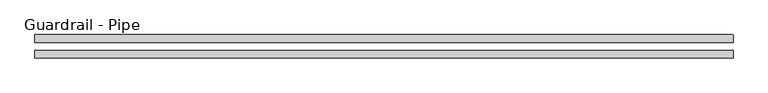
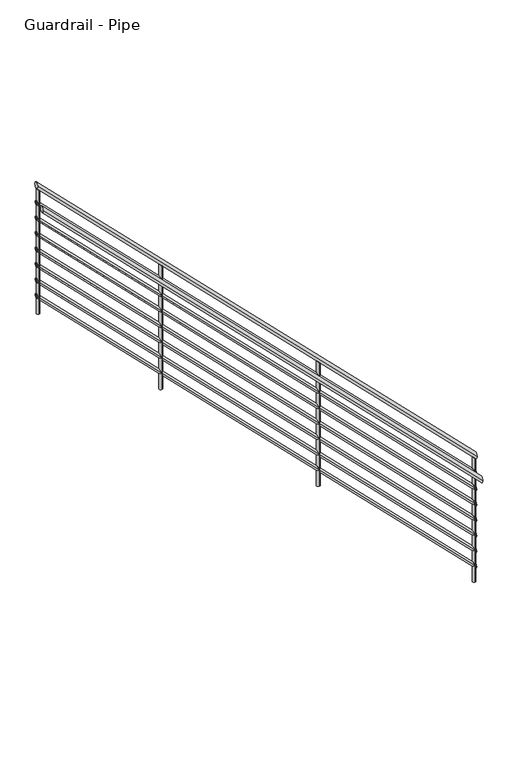
"""IFC4 building model written with IfcOpenShell, lengths in millimetres: railing geometry, Guardrail - Pipe."""

from ifc_helpers import new_model, si_unit, frame, origin, place, context, project, spatial, circle_curve, ellipse_curve, source, transform, mapped, element, save
from ifc_brep_helpers import plane_surface, cylinder_surface, advanced_brep


def guardrail_pipe_ce189c05(model_context):
    return source(origin(), model_context, "Body", "AdvancedBrep", [
        advanced_brep(
        [(-7243.3085296, -3994.9836772, 1268.4592316), (-7243.3085296, -3956.8836772, 1268.4592316), (-10645.1029016, -3994.9836772, 4670.2536037), (-10645.1029016, -3956.8836772, 4670.2536037)],
        [
            (0, 1, ellipse_curve(frame((-7243.3085296, -3975.9336772, 1268.4592316), z_axis=(1.0, 0.0, 0.0), x_axis=(0.0, 0.0, -1.0)), 26.9407684, 19.05)),
            (1, 0, ellipse_curve(frame((-7243.3085296, -3975.9336772, 1268.4592316), z_axis=(1.0, 0.0, 0.0), x_axis=(0.0, 0.0, -1.0)), 26.9407684, 19.05)),
            (2, 3, ellipse_curve(frame((-10645.1029016, -3975.9336772, 4670.2536037), z_axis=(-1.0, 0.0, 0.0), x_axis=(0.0, 0.0, -1.0)), 26.9407684, 19.05)),
            (3, 2, ellipse_curve(frame((-10645.1029016, -3975.9336772, 4670.2536037), z_axis=(-1.0, 0.0, 0.0), x_axis=(0.0, 0.0, -1.0)), 26.9407684, 19.05)),
            (0, 2),
            (3, 1),
        ],
        [
            plane_surface(frame((-7243.3085296, -3975.9336772, 1295.4), z_axis=(1.0, 0.0, 0.0), x_axis=(0.0, -1.0, 0.0))),
            plane_surface(frame((-10645.1029016, -3975.9336772, 4697.194372), z_axis=(-1.0, 0.0, 0.0), x_axis=(0.0, -1.0, 0.0))),
            cylinder_surface(frame((-7256.7789137, -3975.9336772, 1281.9296158), z_axis=(0.7071067811865476, 0.0, -0.7071067811865476), x_axis=(0.0, 1.0, 0.0)), 19.05),
        ],
        [
            (0, [[1, 2]]),
            (1, [[3, 4]]),
            (2, [[-1, 5, -4, 6]]),
            (2, [[-2, -6, -3, -5]]),
        ],
    ),
        advanced_brep(
        [(-7243.3085296, -3988.6336772, 1125.0394878), (-7243.3085296, -3963.2336772, 1125.0394878), (-10645.1029016, -3988.6336772, 4526.8338598), (-10645.1029016, -3963.2336772, 4526.8338598)],
        [
            (0, 1, ellipse_curve(frame((-7243.3085296, -3975.9336772, 1125.0394878), z_axis=(1.0, 0.0, 0.0), x_axis=(0.0, 0.0, -1.0)), 17.9605122, 12.7)),
            (1, 0, ellipse_curve(frame((-7243.3085296, -3975.9336772, 1125.0394878), z_axis=(1.0, 0.0, 0.0), x_axis=(0.0, 0.0, -1.0)), 17.9605122, 12.7)),
            (2, 3, ellipse_curve(frame((-10645.1029016, -3975.9336772, 4526.8338598), z_axis=(-1.0, 0.0, 0.0), x_axis=(0.0, 0.0, -1.0)), 17.9605122, 12.7)),
            (3, 2, ellipse_curve(frame((-10645.1029016, -3975.9336772, 4526.8338598), z_axis=(-1.0, 0.0, 0.0), x_axis=(0.0, 0.0, -1.0)), 17.9605122, 12.7)),
            (0, 2),
            (3, 1),
        ],
        [
            plane_surface(frame((-7243.3085296, -3975.9336772, 1143.0), z_axis=(1.0, 0.0, 0.0), x_axis=(0.0, -1.0, 0.0))),
            plane_surface(frame((-10645.1029016, -3975.9336772, 4544.794372), z_axis=(-1.0, 0.0, 0.0), x_axis=(0.0, -1.0, 0.0))),
            cylinder_surface(frame((-7252.2887857, -3975.9336772, 1134.0197439), z_axis=(0.7071067811865476, 0.0, -0.7071067811865476), x_axis=(0.0, 1.0, 0.0)), 12.7),
        ],
        [
            (0, [[1, 2]]),
            (1, [[3, 4]]),
            (2, [[-1, 5, -4, 6]]),
            (2, [[-2, -6, -3, -5]]),
        ],
    ),
        advanced_brep(
        [(-7243.3085296, -4071.1836772, 1116.0592316), (-7243.3085296, -4033.0836772, 1116.0592316), (-10645.1029016, -4071.1836772, 4517.8536037), (-10645.1029016, -4033.0836772, 4517.8536037)],
        [
            (0, 1, ellipse_curve(frame((-7243.3085296, -4052.1336772, 1116.0592316), z_axis=(1.0, 0.0, 0.0), x_axis=(0.0, 0.0, -1.0)), 26.9407684, 19.05)),
            (1, 0, ellipse_curve(frame((-7243.3085296, -4052.1336772, 1116.0592316), z_axis=(1.0, 0.0, 0.0), x_axis=(0.0, 0.0, -1.0)), 26.9407684, 19.05)),
            (2, 3, ellipse_curve(frame((-10645.1029016, -4052.1336772, 4517.8536037), z_axis=(-1.0, 0.0, 0.0), x_axis=(0.0, 0.0, -1.0)), 26.9407684, 19.05)),
            (3, 2, ellipse_curve(frame((-10645.1029016, -4052.1336772, 4517.8536037), z_axis=(-1.0, 0.0, 0.0), x_axis=(0.0, 0.0, -1.0)), 26.9407684, 19.05)),
            (0, 2),
            (3, 1),
        ],
        [
            plane_surface(frame((-7243.3085296, -4052.1336772, 1143.0), z_axis=(1.0, 0.0, 0.0), x_axis=(0.0, -1.0, 0.0))),
            plane_surface(frame((-10645.1029016, -4052.1336772, 4544.794372), z_axis=(-1.0, 0.0, 0.0), x_axis=(0.0, -1.0, 0.0))),
            cylinder_surface(frame((-7256.7789137, -4052.1336772, 1129.5296158), z_axis=(0.7071067811865476, 0.0, -0.7071067811865476), x_axis=(0.0, 1.0, 0.0)), 19.05),
        ],
        [
            (0, [[1, 2]]),
            (1, [[3, 4]]),
            (2, [[-1, 5, -4, 6]]),
            (2, [[-2, -6, -3, -5]]),
        ],
    ),
        advanced_brep(
        [(-7243.3085296, -3988.6336772, 998.0394878), (-7243.3085296, -3963.2336772, 998.0394878), (-10645.1029016, -3988.6336772, 4399.8338598), (-10645.1029016, -3963.2336772, 4399.8338598)],
        [
            (0, 1, ellipse_curve(frame((-7243.3085296, -3975.9336772, 998.0394878), z_axis=(1.0, 0.0, 0.0), x_axis=(0.0, 0.0, -1.0)), 17.9605122, 12.7)),
            (1, 0, ellipse_curve(frame((-7243.3085296, -3975.9336772, 998.0394878), z_axis=(1.0, 0.0, 0.0), x_axis=(0.0, 0.0, -1.0)), 17.9605122, 12.7)),
            (2, 3, ellipse_curve(frame((-10645.1029016, -3975.9336772, 4399.8338598), z_axis=(-1.0, 0.0, 0.0), x_axis=(0.0, 0.0, -1.0)), 17.9605122, 12.7)),
            (3, 2, ellipse_curve(frame((-10645.1029016, -3975.9336772, 4399.8338598), z_axis=(-1.0, 0.0, 0.0), x_axis=(0.0, 0.0, -1.0)), 17.9605122, 12.7)),
            (0, 2),
            (3, 1),
        ],
        [
            plane_surface(frame((-7243.3085296, -3975.9336772, 1016.0), z_axis=(1.0, 0.0, 0.0), x_axis=(0.0, -1.0, 0.0))),
            plane_surface(frame((-10645.1029016, -3975.9336772, 4417.794372), z_axis=(-1.0, 0.0, 0.0), x_axis=(0.0, -1.0, 0.0))),
            cylinder_surface(frame((-7252.2887857, -3975.9336772, 1007.0197439), z_axis=(0.7071067811865476, 0.0, -0.7071067811865476), x_axis=(0.0, 1.0, 0.0)), 12.7),
        ],
        [
            (0, [[1, 2]]),
            (1, [[3, 4]]),
            (2, [[-1, 5, -4, 6]]),
            (2, [[-2, -6, -3, -5]]),
        ],
    ),
        advanced_brep(
        [(-7243.3085296, -3988.6336772, 871.0394878), (-7243.3085296, -3963.2336772, 871.0394878), (-10645.1029016, -3988.6336772, 4272.8338598), (-10645.1029016, -3963.2336772, 4272.8338598)],
        [
            (0, 1, ellipse_curve(frame((-7243.3085296, -3975.9336772, 871.0394878), z_axis=(1.0, 0.0, 0.0), x_axis=(0.0, 0.0, -1.0)), 17.9605122, 12.7)),
            (1, 0, ellipse_curve(frame((-7243.3085296, -3975.9336772, 871.0394878), z_axis=(1.0, 0.0, 0.0), x_axis=(0.0, 0.0, -1.0)), 17.9605122, 12.7)),
            (2, 3, ellipse_curve(frame((-10645.1029016, -3975.9336772, 4272.8338598), z_axis=(-1.0, 0.0, 0.0), x_axis=(0.0, 0.0, -1.0)), 17.9605122, 12.7)),
            (3, 2, ellipse_curve(frame((-10645.1029016, -3975.9336772, 4272.8338598), z_axis=(-1.0, 0.0, 0.0), x_axis=(0.0, 0.0, -1.0)), 17.9605122, 12.7)),
            (0, 2),
            (3, 1),
        ],
        [
            plane_surface(frame((-7243.3085296, -3975.9336772, 889.0), z_axis=(1.0, 0.0, 0.0), x_axis=(0.0, -1.0, 0.0))),
            plane_surface(frame((-10645.1029016, -3975.9336772, 4290.794372), z_axis=(-1.0, 0.0, 0.0), x_axis=(0.0, -1.0, 0.0))),
            cylinder_surface(frame((-7252.2887857, -3975.9336772, 880.0197439), z_axis=(0.7071067811865476, 0.0, -0.7071067811865476), x_axis=(0.0, 1.0, 0.0)), 12.7),
        ],
        [
            (0, [[1, 2]]),
            (1, [[3, 4]]),
            (2, [[-1, 5, -4, 6]]),
            (2, [[-2, -6, -3, -5]]),
        ],
    ),
        advanced_brep(
        [(-7243.3085296, -3988.6336772, 744.0394878), (-7243.3085296, -3963.2336772, 744.0394878), (-10645.1029016, -3988.6336772, 4145.8338598), (-10645.1029016, -3963.2336772, 4145.8338598)],
        [
            (0, 1, ellipse_curve(frame((-7243.3085296, -3975.9336772, 744.0394878), z_axis=(1.0, 0.0, 0.0), x_axis=(0.0, 0.0, -1.0)), 17.9605122, 12.7)),
            (1, 0, ellipse_curve(frame((-7243.3085296, -3975.9336772, 744.0394878), z_axis=(1.0, 0.0, 0.0), x_axis=(0.0, 0.0, -1.0)), 17.9605122, 12.7)),
            (2, 3, ellipse_curve(frame((-10645.1029016, -3975.9336772, 4145.8338598), z_axis=(-1.0, 0.0, 0.0), x_axis=(0.0, 0.0, -1.0)), 17.9605122, 12.7)),
            (3, 2, ellipse_curve(frame((-10645.1029016, -3975.9336772, 4145.8338598), z_axis=(-1.0, 0.0, 0.0), x_axis=(0.0, 0.0, -1.0)), 17.9605122, 12.7)),
            (0, 2),
            (3, 1),
        ],
        [
            plane_surface(frame((-7243.3085296, -3975.9336772, 762.0), z_axis=(1.0, 0.0, 0.0), x_axis=(0.0, -1.0, 0.0))),
            plane_surface(frame((-10645.1029016, -3975.9336772, 4163.794372), z_axis=(-1.0, 0.0, 0.0), x_axis=(0.0, -1.0, 0.0))),
            cylinder_surface(frame((-7252.2887857, -3975.9336772, 753.0197439), z_axis=(0.7071067811865476, 0.0, -0.7071067811865476), x_axis=(0.0, 1.0, 0.0)), 12.7),
        ],
        [
            (0, [[1, 2]]),
            (1, [[3, 4]]),
            (2, [[-1, 5, -4, 6]]),
            (2, [[-2, -6, -3, -5]]),
        ],
    ),
        advanced_brep(
        [(-7243.3085296, -3988.6336772, 617.0394878), (-7243.3085296, -3963.2336772, 617.0394878), (-10645.1029016, -3988.6336772, 4018.8338598), (-10645.1029016, -3963.2336772, 4018.8338598)],
        [
            (0, 1, ellipse_curve(frame((-7243.3085296, -3975.9336772, 617.0394878), z_axis=(1.0, 0.0, 0.0), x_axis=(0.0, 0.0, -1.0)), 17.9605122, 12.7)),
            (1, 0, ellipse_curve(frame((-7243.3085296, -3975.9336772, 617.0394878), z_axis=(1.0, 0.0, 0.0), x_axis=(0.0, 0.0, -1.0)), 17.9605122, 12.7)),
            (2, 3, ellipse_curve(frame((-10645.1029016, -3975.9336772, 4018.8338598), z_axis=(-1.0, 0.0, 0.0), x_axis=(0.0, 0.0, -1.0)), 17.9605122, 12.7)),
            (3, 2, ellipse_curve(frame((-10645.1029016, -3975.9336772, 4018.8338598), z_axis=(-1.0, 0.0, 0.0), x_axis=(0.0, 0.0, -1.0)), 17.9605122, 12.7)),
            (0, 2),
            (3, 1),
        ],
        [
            plane_surface(frame((-7243.3085296, -3975.9336772, 635.0), z_axis=(1.0, 0.0, 0.0), x_axis=(0.0, -1.0, 0.0))),
            plane_surface(frame((-10645.1029016, -3975.9336772, 4036.794372), z_axis=(-1.0, 0.0, 0.0), x_axis=(0.0, -1.0, 0.0))),
            cylinder_surface(frame((-7252.2887857, -3975.9336772, 626.0197439), z_axis=(0.7071067811865476, 0.0, -0.7071067811865476), x_axis=(0.0, 1.0, 0.0)), 12.7),
        ],
        [
            (0, [[1, 2]]),
            (1, [[3, 4]]),
            (2, [[-1, 5, -4, 6]]),
            (2, [[-2, -6, -3, -5]]),
        ],
    ),
        advanced_brep(
        [(-7243.3085296, -3988.6336772, 490.0394878), (-7243.3085296, -3963.2336772, 490.0394878), (-10645.1029016, -3988.6336772, 3891.8338598), (-10645.1029016, -3963.2336772, 3891.8338598)],
        [
            (0, 1, ellipse_curve(frame((-7243.3085296, -3975.9336772, 490.0394878), z_axis=(1.0, 0.0, 0.0), x_axis=(0.0, 0.0, -1.0)), 17.9605122, 12.7)),
            (1, 0, ellipse_curve(frame((-7243.3085296, -3975.9336772, 490.0394878), z_axis=(1.0, 0.0, 0.0), x_axis=(0.0, 0.0, -1.0)), 17.9605122, 12.7)),
            (2, 3, ellipse_curve(frame((-10645.1029016, -3975.9336772, 3891.8338598), z_axis=(-1.0, 0.0, 0.0), x_axis=(0.0, 0.0, -1.0)), 17.9605122, 12.7)),
            (3, 2, ellipse_curve(frame((-10645.1029016, -3975.9336772, 3891.8338598), z_axis=(-1.0, 0.0, 0.0), x_axis=(0.0, 0.0, -1.0)), 17.9605122, 12.7)),
            (0, 2),
            (3, 1),
        ],
        [
            plane_surface(frame((-7243.3085296, -3975.9336772, 508.0), z_axis=(1.0, 0.0, 0.0), x_axis=(0.0, -1.0, 0.0))),
            plane_surface(frame((-10645.1029016, -3975.9336772, 3909.794372), z_axis=(-1.0, 0.0, 0.0), x_axis=(0.0, -1.0, 0.0))),
            cylinder_surface(frame((-7252.2887857, -3975.9336772, 499.0197439), z_axis=(0.7071067811865476, 0.0, -0.7071067811865476), x_axis=(0.0, 1.0, 0.0)), 12.7),
        ],
        [
            (0, [[1, 2]]),
            (1, [[3, 4]]),
            (2, [[-1, 5, -4, 6]]),
            (2, [[-2, -6, -3, -5]]),
        ],
    ),
        advanced_brep(
        [(-7243.3085296, -3988.6336772, 363.0394878), (-7243.3085296, -3963.2336772, 363.0394878), (-10645.1029016, -3988.6336772, 3764.8338598), (-10645.1029016, -3963.2336772, 3764.8338598)],
        [
            (0, 1, ellipse_curve(frame((-7243.3085296, -3975.9336772, 363.0394878), z_axis=(1.0, 0.0, 0.0), x_axis=(0.0, 0.0, -1.0)), 17.9605122, 12.7)),
            (1, 0, ellipse_curve(frame((-7243.3085296, -3975.9336772, 363.0394878), z_axis=(1.0, 0.0, 0.0), x_axis=(0.0, 0.0, -1.0)), 17.9605122, 12.7)),
            (2, 3, ellipse_curve(frame((-10645.1029016, -3975.9336772, 3764.8338598), z_axis=(-1.0, 0.0, 0.0), x_axis=(0.0, 0.0, -1.0)), 17.9605122, 12.7)),
            (3, 2, ellipse_curve(frame((-10645.1029016, -3975.9336772, 3764.8338598), z_axis=(-1.0, 0.0, 0.0), x_axis=(0.0, 0.0, -1.0)), 17.9605122, 12.7)),
            (0, 2),
            (3, 1),
        ],
        [
            plane_surface(frame((-7243.3085296, -3975.9336772, 381.0), z_axis=(1.0, 0.0, 0.0), x_axis=(0.0, -1.0, 0.0))),
            plane_surface(frame((-10645.1029016, -3975.9336772, 3782.794372), z_axis=(-1.0, 0.0, 0.0), x_axis=(0.0, -1.0, 0.0))),
            cylinder_surface(frame((-7252.2887857, -3975.9336772, 372.0197439), z_axis=(0.7071067811865476, 0.0, -0.7071067811865476), x_axis=(0.0, 1.0, 0.0)), 12.7),
        ],
        [
            (0, [[1, 2]]),
            (1, [[3, 4]]),
            (2, [[-1, 5, -4, 6]]),
            (2, [[-2, -6, -3, -5]]),
        ],
    ),
        advanced_brep(
        [(-9681.7085296, -3963.2336772, 3679.9184633), (-9681.7085296, -3963.2336772, 2667.0), (-9681.7085296, -3988.6336772, 2667.0), (-9681.7085296, -3988.6336772, 3679.9184633)],
        [
            (0, 1),
            (1, 2, circle_curve(frame((-9681.7085296, -3975.9336772, 2667.0), z_axis=(0.0, 0.0, 1.0), x_axis=(0.0, -1.0, 0.0)), 12.7)),
            (2, 3),
            (3, 0, ellipse_curve(frame((-9681.7085296, -3975.9336772, 3679.9184633), z_axis=(-0.7071067811865471, 0.0, -0.7071067811865479), x_axis=(-0.7071067811865479, 0.0, 0.7071067811865471)), 17.9605122, 12.7)),
            (0, 3, ellipse_curve(frame((-9681.7085296, -3975.9336772, 3679.9184633), z_axis=(-0.7071067811865471, 0.0, -0.7071067811865479), x_axis=(-0.7071067811865479, 0.0, 0.7071067811865471)), 17.9605122, 12.7)),
            (2, 1, circle_curve(frame((-9681.7085296, -3975.9336772, 2667.0), z_axis=(0.0, 0.0, 1.0), x_axis=(0.0, -1.0, 0.0)), 12.7)),
        ],
        [
            cylinder_surface(frame((-9681.7085296, -3975.9336772, 2438.4), z_axis=(0.0, 0.0, 1.0), x_axis=(0.0, -1.0, 0.0)), 12.7),
            plane_surface(frame((-9707.1085296, -4001.3336772, 3705.3184633), z_axis=(0.7071067811865471, 0.0, 0.7071067811865479), x_axis=(0.0, 1.0, 0.0))),
            plane_surface(frame((-9656.3085296, -4001.3336772, 2667.0), z_axis=(0.0, 0.0, -1.0), x_axis=(0.0, 1.0, 0.0))),
        ],
        [
            (0, [[1, 2, 3, 4]]),
            (0, [[-1, 5, -3, 6]]),
            (1, [[-4, -5]]),
            (2, [[-2, -6]]),
        ],
    ),
        advanced_brep(
        [(-8462.5085296, -3963.2336772, 2460.7184633), (-8462.5085296, -3963.2336772, 1447.8), (-8462.5085296, -3988.6336772, 1447.8), (-8462.5085296, -3988.6336772, 2460.7184633)],
        [
            (0, 1),
            (1, 2, circle_curve(frame((-8462.5085296, -3975.9336772, 1447.8), z_axis=(0.0, 0.0, 1.0), x_axis=(0.0, -1.0, 0.0)), 12.7)),
            (2, 3),
            (3, 0, ellipse_curve(frame((-8462.5085296, -3975.9336772, 2460.7184633), z_axis=(-0.7071067811865471, 0.0, -0.7071067811865479), x_axis=(-0.7071067811865479, 0.0, 0.7071067811865471)), 17.9605122, 12.7)),
            (0, 3, ellipse_curve(frame((-8462.5085296, -3975.9336772, 2460.7184633), z_axis=(-0.7071067811865471, 0.0, -0.7071067811865479), x_axis=(-0.7071067811865479, 0.0, 0.7071067811865471)), 17.9605122, 12.7)),
            (2, 1, circle_curve(frame((-8462.5085296, -3975.9336772, 1447.8), z_axis=(0.0, 0.0, 1.0), x_axis=(0.0, -1.0, 0.0)), 12.7)),
        ],
        [
            cylinder_surface(frame((-8462.5085296, -3975.9336772, 1219.2), z_axis=(0.0, 0.0, 1.0), x_axis=(0.0, -1.0, 0.0)), 12.7),
            plane_surface(frame((-8487.9085296, -4001.3336772, 2486.1184633), z_axis=(0.7071067811865471, 0.0, 0.7071067811865479), x_axis=(0.0, 1.0, 0.0))),
            plane_surface(frame((-8437.1085296, -4001.3336772, 1447.8), z_axis=(0.0, 0.0, -1.0), x_axis=(0.0, 1.0, 0.0))),
        ],
        [
            (0, [[1, 2, 3, 4]]),
            (0, [[-1, 5, -3, 6]]),
            (1, [[-4, -5]]),
            (2, [[-2, -6]]),
        ],
    ),
        advanced_brep(
        [(-10632.4029016, -3963.2336772, 4630.6128353), (-10632.4029016, -3963.2336772, 3617.694372), (-10632.4029016, -3988.6336772, 3617.694372), (-10632.4029016, -3988.6336772, 4630.6128353)],
        [
            (0, 1),
            (1, 2, circle_curve(frame((-10632.4029016, -3975.9336772, 3617.694372), z_axis=(0.0, 0.0, 1.0), x_axis=(0.0, -1.0, 0.0)), 12.7)),
            (2, 3),
            (3, 0, ellipse_curve(frame((-10632.4029016, -3975.9336772, 4630.6128353), z_axis=(-0.7071067811865471, 0.0, -0.7071067811865479), x_axis=(-0.7071067811865479, 0.0, 0.7071067811865471)), 17.9605122, 12.7)),
            (0, 3, ellipse_curve(frame((-10632.4029016, -3975.9336772, 4630.6128353), z_axis=(-0.7071067811865471, 0.0, -0.7071067811865479), x_axis=(-0.7071067811865479, 0.0, 0.7071067811865471)), 17.9605122, 12.7)),
            (2, 1, circle_curve(frame((-10632.4029016, -3975.9336772, 3617.694372), z_axis=(0.0, 0.0, 1.0), x_axis=(0.0, -1.0, 0.0)), 12.7)),
        ],
        [
            cylinder_surface(frame((-10632.4029016, -3975.9336772, 3389.094372), z_axis=(0.0, 0.0, 1.0), x_axis=(0.0, -1.0, 0.0)), 12.7),
            plane_surface(frame((-10657.8029016, -4001.3336772, 4656.0128353), z_axis=(0.7071067811865471, 0.0, 0.7071067811865479), x_axis=(0.0, 1.0, 0.0))),
            plane_surface(frame((-10607.0029016, -4001.3336772, 3617.694372), z_axis=(0.0, 0.0, -1.0), x_axis=(0.0, 1.0, 0.0))),
        ],
        [
            (0, [[1, 2, 3, 4]]),
            (0, [[-1, 5, -3, 6]]),
            (1, [[-4, -5]]),
            (2, [[-2, -6]]),
        ],
    ),
        advanced_brep(
        [(-7256.0085296, -3963.2336772, 1254.2184633), (-7256.0085296, -3963.2336772, 241.3), (-7256.0085296, -3988.6336772, 241.3), (-7256.0085296, -3988.6336772, 1254.2184633)],
        [
            (0, 1),
            (1, 2, circle_curve(frame((-7256.0085296, -3975.9336772, 241.3), z_axis=(0.0, 0.0, 1.0), x_axis=(0.0, -1.0, 0.0)), 12.7)),
            (2, 3),
            (3, 0, ellipse_curve(frame((-7256.0085296, -3975.9336772, 1254.2184633), z_axis=(-0.7071067811865471, 0.0, -0.7071067811865479), x_axis=(-0.7071067811865479, 0.0, 0.7071067811865471)), 17.9605122, 12.7)),
            (0, 3, ellipse_curve(frame((-7256.0085296, -3975.9336772, 1254.2184633), z_axis=(-0.7071067811865471, 0.0, -0.7071067811865479), x_axis=(-0.7071067811865479, 0.0, 0.7071067811865471)), 17.9605122, 12.7)),
            (2, 1, circle_curve(frame((-7256.0085296, -3975.9336772, 241.3), z_axis=(0.0, 0.0, 1.0), x_axis=(0.0, -1.0, 0.0)), 12.7)),
        ],
        [
            cylinder_surface(frame((-7256.0085296, -3975.9336772, 12.7), z_axis=(0.0, 0.0, 1.0), x_axis=(0.0, -1.0, 0.0)), 12.7),
            plane_surface(frame((-7281.4085296, -4001.3336772, 1279.6184633), z_axis=(0.7071067811865471, 0.0, 0.7071067811865479), x_axis=(0.0, 1.0, 0.0))),
            plane_surface(frame((-7230.6085296, -4001.3336772, 241.3), z_axis=(0.0, 0.0, -1.0), x_axis=(0.0, 1.0, 0.0))),
        ],
        [
            (0, [[1, 2, 3, 4]]),
            (0, [[-1, 5, -3, 6]]),
            (1, [[-4, -5]]),
            (2, [[-2, -6]]),
        ],
    ),
    ])


if __name__ == "__main__":
    model = new_model("IFC4")
    model_context = context("Model", 3, world=origin())
    ifc_project = project(units=[si_unit("LENGTHUNIT", "METRE", prefix="MILLI")], contexts=[model_context])
    site = spatial("IfcSite", under=ifc_project)
    building = spatial("IfcBuilding", under=site)
    placement = place(None, origin())
    guardrail_pipe_shape = guardrail_pipe_ce189c05(model_context)
    element("IfcRailing", 1, ObjectType="Guardrail - Pipe", at=placement, inside=building, context=model_context, shape_type="MappedRepresentation", body=[
        mapped(guardrail_pipe_shape, transform((0.0, 0.0, 0.0), x_axis=(1.0, 0.0, 0.0), y_axis=(0.0, 1.0, 0.0), z_axis=(0.0, 0.0, 1.0))),
    ])
    save(model, "model.ifc")

# Revit data of these elements
# Element 1 (IfcRailing, "Guardrail - Pipe")
#   Materials on its faces: "Plastic - Vinyl Cove Base"
# Materials
#   "Plastic - Vinyl Cove Base": class "Plastic", colour RGB 5 5 5, transparency 0, Cost = 0
